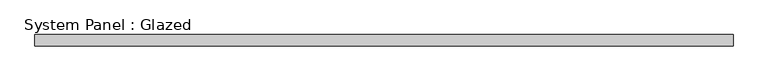
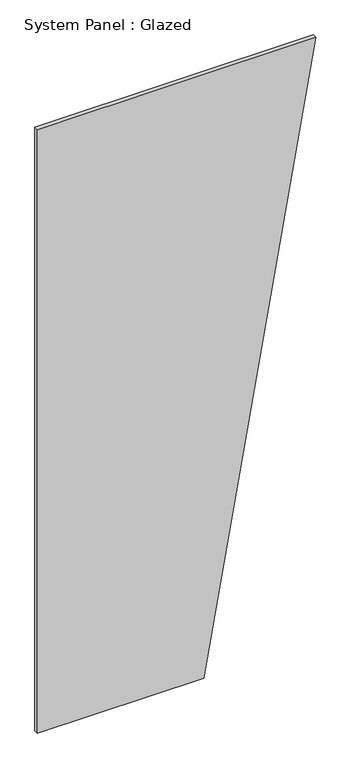
"""IFC4 building model written with IfcOpenShell, lengths in millimetres: plate geometry, System Panel : Glazed."""

from ifc_helpers import new_model, si_unit, frame, origin, place, context, project, spatial, polyline, outline, extrude, source, transform, mapped, element, save


def system_panel_glazed_2bad594a(model_context):
    return source(origin(), model_context, "Body", "SweptSolid", [
        extrude(outline(polyline([(0.0, -797.3917397), (0.0, 154.912342), (3657.6, 797.3917397), (3657.6, -797.3917397), (0.0, -797.3917397)])), frame((0.0, -44.45, 0.0), z_axis=(0.0, 1.0, 0.0), x_axis=(0.0, 0.0, 1.0)), (0.0, 0.0, 1.0), 25.4),
    ])


if __name__ == "__main__":
    model = new_model("IFC4")
    model_context = context("Model", 3, world=origin())
    ifc_project = project(units=[si_unit("LENGTHUNIT", "METRE", prefix="MILLI")], contexts=[model_context])
    site = spatial("IfcSite", under=ifc_project)
    building = spatial("IfcBuilding", under=site)
    placement = place(None, origin())
    system_panel_glazed_shape = system_panel_glazed_2bad594a(model_context)
    element("IfcPlate", 1, ObjectType="System Panel : Glazed", at=placement, inside=building, context=model_context, shape_type="MappedRepresentation", body=[
        mapped(system_panel_glazed_shape, transform((0.0, 0.0, 0.0), x_axis=(1.0, 0.0, 0.0), y_axis=(0.0, 1.0, 0.0), z_axis=(0.0, 0.0, 1.0))),
    ])
    save(model, "model.ifc")

# Revit data of these elements
# Type "System Panel : Glazed"
#   Construction Type Id = "GSP4R"
#   Analytic Construction = "1/8 in Pilkington single glazing"
#   Visual Light Transmittance = 0.9
#   Solar Heat Gain Coefficient = 0.86
#   Heat Transfer Coefficient (U) = 1.18115 BTU/(h·ft²·°F)
#   Define Thermal Properties by = 1
# Element 1 (IfcPlate, "System Panel : Glazed")
#   Materials on its faces: "Glass"
# Materials
#   "Glass": class "Glass", colour RGB 0 128 192, transparency 0.75, Description = "Soda Lime Glass", Cost = 0
